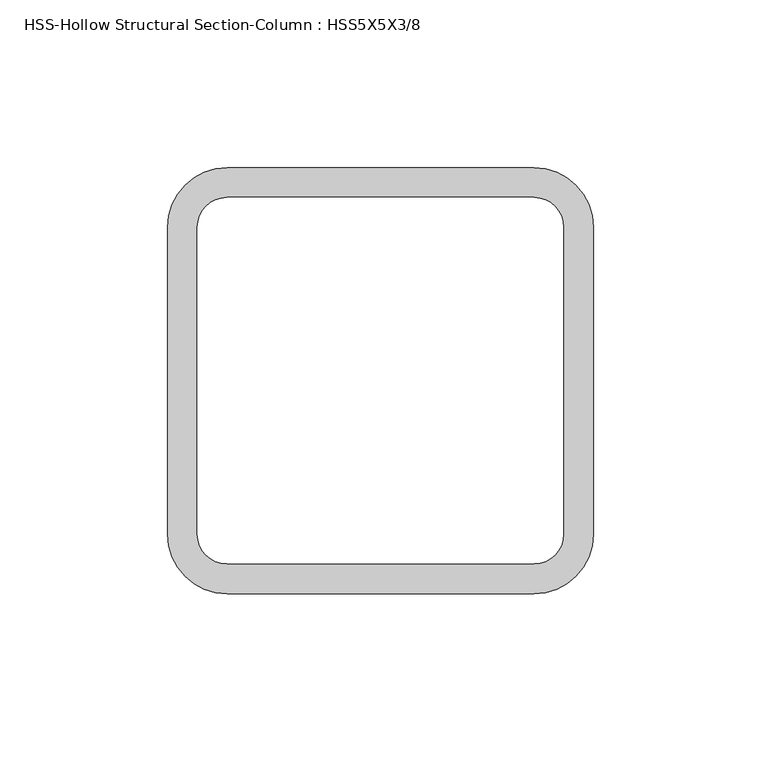
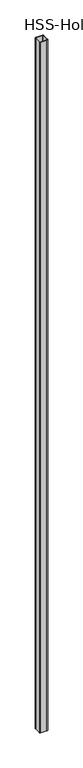
"""IFC4 building model written with IfcOpenShell, lengths in millimetres: column geometry, HSS-Hollow Structural Section-Column : HSS5X5X3/8."""

import ifcopenshell
import ifcopenshell.guid

model = None  # the IFC model being written
_history = None  # IfcOwnerHistory: only IFC2X3 demands one
_inside = {}  # id of a spatial element -> (the spatial element, [elements in it])
_under = {}  # id of a project, library or spatial element -> (it, [spatial elements below it])
_declared = {}  # id of a project -> (the project, [libraries it declares])
_typed = {}  # id of a type object -> (the type object, [elements of that type])
_made_of = {}  # id of a material, layer set ... -> (it, [elements and type objects made of it])


def new_model(schema):
    """Start an empty IFC model of exactly this schema.

    Asked for "IFC4X3", IfcOpenShell would pick the latest addendum, in which some entities
    have other attributes; the version numbers below select the first issue.
    IFC2X3 requires an IfcOwnerHistory on every rooted entity: one is made here for all.
    """
    global model, _history
    if schema == "IFC4X3":
        model = ifcopenshell.file(schema_version=(4, 3, 0, 0))
    else:
        model = ifcopenshell.file(schema=schema)
    _inside.clear()
    _under.clear()
    _declared.clear()
    _typed.clear()
    _made_of.clear()
    _history = None
    if model.schema == "IFC2X3":
        org = make("IfcOrganization", Name="unknown")
        user = make(
            "IfcPersonAndOrganization",
            ThePerson=make("IfcPerson", FamilyName="unknown"),
            TheOrganization=org,
        )
        app = make(
            "IfcApplication",
            ApplicationDeveloper=org,
            Version="unknown",
            ApplicationFullName="unknown",
            ApplicationIdentifier="unknown",
        )
        _history = make(
            "IfcOwnerHistory",
            OwningUser=user,
            OwningApplication=app,
            ChangeAction="ADDED",
            CreationDate=0,
        )
    return model


def make(cls, **values):
    """One entity of the class cls with the attributes given. An attribute that is None is left unset."""
    return model.create_entity(
        cls, **{name: value for name, value in values.items() if value is not None}
    )


def rooted(cls, **values):
    """An entity with a GlobalId (a new one), such as an element, a storey or a relation."""
    return make(cls, GlobalId=ifcopenshell.guid.new(), OwnerHistory=_history, **values)


def si_unit(unit_type, name, prefix=None):
    """IfcSIUnit, for example si_unit("LENGTHUNIT", "METRE", prefix="MILLI")."""
    return make("IfcSIUnit", UnitType=unit_type, Prefix=prefix, Name=name)


def assignment(units):
    """IfcUnitAssignment: the units of a project."""
    return None if units is None else make("IfcUnitAssignment", Units=units)


def point(xyz):
    """IfcCartesianPoint."""
    return None if xyz is None else make("IfcCartesianPoint", Coordinates=xyz)


def direction(xyz):
    """IfcDirection."""
    return None if xyz is None else make("IfcDirection", DirectionRatios=xyz)


def frame(location, z_axis=None, x_axis=None):
    """IfcAxis2Placement3D, a coordinate frame: its origin and axes. An axis left out is left unset."""
    return make(
        "IfcAxis2Placement3D",
        Location=point(location),
        Axis=direction(z_axis),
        RefDirection=direction(x_axis),
    )


def frame_2d(location, x_axis=None):
    """IfcAxis2Placement2D, a coordinate frame in the plane: its origin and x axis."""
    return make(
        "IfcAxis2Placement2D", Location=point(location), RefDirection=direction(x_axis)
    )


def origin():
    """The frame at (0, 0, 0) with its axes left unset."""
    return frame((0.0, 0.0, 0.0))


def place(relative_to, where):
    """IfcLocalPlacement: puts the frame where relative to a parent placement (None: the world)."""
    return make(
        "IfcLocalPlacement", PlacementRelTo=relative_to, RelativePlacement=where
    )


def context(
    kind, dimensions, precision=None, world=None, true_north=None, identifier=None
):
    """IfcGeometricRepresentationContext, for example the 3D "Model" context."""
    return make(
        "IfcGeometricRepresentationContext",
        ContextIdentifier=identifier,
        ContextType=kind,
        CoordinateSpaceDimension=dimensions,
        Precision=precision,
        WorldCoordinateSystem=world,
        TrueNorth=true_north,
    )


def project(units=None, contexts=None):
    """IfcProject with its units and contexts."""
    return rooted(
        "IfcProject",
        Name="project",
        RepresentationContexts=contexts,
        UnitsInContext=assignment(units),
    )


def spatial(cls, under=None, at=None, **own):
    """A site, building, storey or space (cls), placed at a placement, below another one or the project."""
    s = rooted(cls, ObjectPlacement=at, **own)
    if under is not None:
        _under.setdefault(under.id(), (under, []))[1].append(s)
    return s


def polyline(points):
    """IfcPolyline through the points."""
    return make("IfcPolyline", Points=[point(p) for p in points])


def circle_curve(where, radius):
    """IfcCircle in the frame where."""
    return make("IfcCircle", Position=where, Radius=radius)


def trimmed(basis, trim1, trim2, sense, master):
    """IfcTrimmedCurve: the piece of a basis curve between two trims."""
    return make(
        "IfcTrimmedCurve",
        BasisCurve=basis,
        Trim1=trim1,
        Trim2=trim2,
        SenseAgreement=sense,
        MasterRepresentation=master,
    )


def segment(curve, same_sense, transition):
    """IfcCompositeCurveSegment."""
    return make(
        "IfcCompositeCurveSegment",
        Transition=transition,
        SameSense=same_sense,
        ParentCurve=curve,
    )


def composite_curve(segments, self_intersect=None):
    """IfcCompositeCurve: segments joined end to end."""
    return make("IfcCompositeCurve", Segments=segments, SelfIntersect=self_intersect)


def outline(outer, holes=None, kind="AREA"):
    """IfcArbitraryClosedProfileDef: a profile drawn as a closed curve; with holes, ...WithVoids."""
    if holes is None:
        return make("IfcArbitraryClosedProfileDef", ProfileType=kind, OuterCurve=outer)
    return make(
        "IfcArbitraryProfileDefWithVoids",
        ProfileType=kind,
        OuterCurve=outer,
        InnerCurves=holes,
    )


def extrude(swept, where, along, depth):
    """IfcExtrudedAreaSolid: the profile swept, set in the frame where, extruded along a direction by depth."""
    return make(
        "IfcExtrudedAreaSolid",
        SweptArea=swept,
        Position=where,
        ExtrudedDirection=direction(along),
        Depth=depth,
    )


def shape(context_of_items, identifier, shape_type, items):
    """IfcShapeRepresentation: the items that make up one representation, for example the "Body"."""
    return make(
        "IfcShapeRepresentation",
        ContextOfItems=context_of_items,
        RepresentationIdentifier=identifier,
        RepresentationType=shape_type,
        Items=items,
    )


def source(mapping_origin, context_of_items, identifier, shape_type, items):
    """IfcRepresentationMap: a shape defined once, which mapped items show again and again."""
    return make(
        "IfcRepresentationMap",
        MappingOrigin=mapping_origin,
        MappedRepresentation=shape(context_of_items, identifier, shape_type, items),
    )


def transform(
    local_origin,
    x_axis=None,
    y_axis=None,
    z_axis=None,
    scale=None,
    scale2=None,
    scale3=None,
    uniform=True,
):
    """IfcCartesianTransformationOperator3D, or its non-uniform kind. x_axis, y_axis, z_axis: its Axis1, 2, 3."""
    if uniform:
        return make(
            "IfcCartesianTransformationOperator3D",
            Axis1=direction(x_axis),
            Axis2=direction(y_axis),
            LocalOrigin=point(local_origin),
            Scale=scale,
            Axis3=direction(z_axis),
        )
    return make(
        "IfcCartesianTransformationOperator3DnonUniform",
        Axis1=direction(x_axis),
        Axis2=direction(y_axis),
        LocalOrigin=point(local_origin),
        Scale=scale,
        Axis3=direction(z_axis),
        Scale2=scale2,
        Scale3=scale3,
    )


def mapped(mapping_source, mapping_target):
    """IfcMappedItem: shows the shape of a source again, moved by a transform."""
    return make(
        "IfcMappedItem", MappingSource=mapping_source, MappingTarget=mapping_target
    )


def made_of(thing, what):
    """Note that an element or type object is made of a material, layer set ...; save() writes the relation."""
    if what is not None:
        _made_of.setdefault(what.id(), (what, []))[1].append(thing)
    return thing


def element(
    cls,
    number,
    at=None,
    inside=None,
    cuts=None,
    type_object=None,
    material=None,
    context=None,
    identifier="Body",
    shape_type=None,
    held_by="IfcProductDefinitionShape",
    body=None,
    shapes=None,
    **own,
):
    """One element of the class cls, such as IfcWall. Its Tag is "e" and its number.

    at: its placement. inside: the storey or other place that contains it. cuts: it is an
    opening in that element (IfcRelVoidsElement). A single representation is given by context,
    identifier, shape_type and body (its items); several are given by shapes. held_by: the class
    of the entity that holds the representations. save() writes the other relations.
    """
    e = rooted(cls, Tag="e%d" % number, ObjectPlacement=at, **own)
    if body is not None:
        shapes = [shape(context, identifier, shape_type, body)]
    if shapes is not None:
        e.Representation = make(held_by, Representations=shapes)
    if inside is not None:
        _inside.setdefault(inside.id(), (inside, []))[1].append(e)
    if cuts is not None:
        rooted(
            "IfcRelVoidsElement", RelatingBuildingElement=cuts, RelatedOpeningElement=e
        )
    if type_object is not None:
        _typed.setdefault(type_object.id(), (type_object, []))[1].append(e)
    return made_of(e, material)


def aggregate(whole, parts):
    """IfcRelAggregates: a whole, such as a stair, and the parts it consists of."""
    return rooted("IfcRelAggregates", RelatingObject=whole, RelatedObjects=parts)


def save(model, path):
    """Write the relations noted so far, then the file.

    IfcRelAggregates (storeys below a building ...), IfcRelContainedInSpatialStructure (elements
    in a storey), IfcRelDefinesByType, IfcRelAssociatesMaterial and IfcRelDeclares: one each for
    every whole, place, type object, material and project.
    """
    for whole, parts in _under.values():
        aggregate(whole, parts)
    for where, things in _inside.values():
        rooted(
            "IfcRelContainedInSpatialStructure",
            RelatedElements=things,
            RelatingStructure=where,
        )
    for kind, things in _typed.values():
        rooted("IfcRelDefinesByType", RelatedObjects=things, RelatingType=kind)
    for what, things in _made_of.values():
        rooted("IfcRelAssociatesMaterial", RelatedObjects=things, RelatingMaterial=what)
    for by, libraries in _declared.values():
        rooted("IfcRelDeclares", RelatingContext=by, RelatedDefinitions=libraries)
    model.write(path)


def hss_hollow_structural_section_column_hss5x5x3_8_a8b47676(model_context):
    return source(origin(), model_context, "Body", "SweptSolid", [
        extrude(outline(composite_curve([segment(trimmed(circle_curve(frame_2d((45.7708, 45.7708)), 17.7292), [point((45.7708, 63.5))], [point((63.5, 45.7708))], False, "CARTESIAN"), True, "CONTINUOUS"), segment(polyline([(63.5, 45.7708), (63.5, -45.7708)]), True, "CONTINUOUS"), segment(trimmed(circle_curve(frame_2d((45.7708, -45.7708)), 17.7292), [point((63.5, -45.7708))], [point((45.7708, -63.5))], False, "CARTESIAN"), True, "CONTINUOUS"), segment(polyline([(45.7708, -63.5), (-45.7708, -63.5)]), True, "CONTINUOUS"), segment(trimmed(circle_curve(frame_2d((-45.7708, -45.7708)), 17.7292), [point((-45.7708, -63.5))], [point((-63.5, -45.7708))], False, "CARTESIAN"), True, "CONTINUOUS"), segment(polyline([(-63.5, -45.7708), (-63.5, 45.7708)]), True, "CONTINUOUS"), segment(trimmed(circle_curve(frame_2d((-45.7708, 45.7708)), 17.7292), [point((-63.5, 45.7708))], [point((-45.7708, 63.5))], False, "CARTESIAN"), True, "CONTINUOUS"), segment(polyline([(-45.7708, 63.5), (45.7708, 63.5)]), True, "CONTINUOUS")], self_intersect=False), holes=[composite_curve([segment(polyline([(45.7708, 54.6354), (-45.7708, 54.6354)]), True, "CONTINUOUS"), segment(trimmed(circle_curve(frame_2d((-45.7708, 45.7708)), 8.8646), [point((-45.7708, 54.6354))], [point((-54.6354, 45.7708))], True, "CARTESIAN"), True, "CONTINUOUS"), segment(polyline([(-54.6354, 45.7708), (-54.6354, -45.7708)]), True, "CONTINUOUS"), segment(trimmed(circle_curve(frame_2d((-45.7708, -45.7708)), 8.8646), [point((-54.6354, -45.7708))], [point((-45.7708, -54.6354))], True, "CARTESIAN"), True, "CONTINUOUS"), segment(polyline([(-45.7708, -54.6354), (45.7708, -54.6354)]), True, "CONTINUOUS"), segment(trimmed(circle_curve(frame_2d((45.7708, -45.7708)), 8.8646), [point((45.7708, -54.6354))], [point((54.6354, -45.7708))], True, "CARTESIAN"), True, "CONTINUOUS"), segment(polyline([(54.6354, -45.7708), (54.6354, 45.7708)]), True, "CONTINUOUS"), segment(trimmed(circle_curve(frame_2d((45.7708, 45.7708)), 8.8646), [point((54.6354, 45.7708))], [point((45.7708, 54.6354))], True, "CARTESIAN"), True, "CONTINUOUS")], self_intersect=False)]), frame((0.0, 0.0, 16408.4), z_axis=(0.0, 0.0, 1.0), x_axis=(1.0, 0.0, 0.0)), (0.0, 0.0, 1.0), 11176.0),
    ])


if __name__ == "__main__":
    model = new_model("IFC4")
    model_context = context("Model", 3, world=origin())
    ifc_project = project(units=[si_unit("LENGTHUNIT", "METRE", prefix="MILLI")], contexts=[model_context])
    site = spatial("IfcSite", under=ifc_project)
    building = spatial("IfcBuilding", under=site)
    placement = place(None, origin())
    hss_hollow_structural_section_column_hss5x5x3_8_shape = hss_hollow_structural_section_column_hss5x5x3_8_a8b47676(model_context)
    element("IfcColumn", 1, ObjectType="HSS-Hollow Structural Section-Column : HSS5X5X3/8", at=placement, inside=building, context=model_context, shape_type="MappedRepresentation", body=[
        mapped(hss_hollow_structural_section_column_hss5x5x3_8_shape, transform((0.0, 0.0, 0.0), x_axis=(1.0, 0.0, 0.0), y_axis=(0.0, 1.0, 0.0), z_axis=(0.0, 0.0, 1.0))),
    ])
    save(model, "model.ifc")

# Revit data of these elements
# Type "HSS-Hollow Structural Section-Column : HSS5X5X3/8"
#   Assembly Code = "B10"
#   Shape = "Square"
#   W = 22.3
#   Ht = 0' - 5"
#   b = 0' - 5"
#   kr = 0' - 0.698"
#   t = 0' - 0.349"
#   A = 0.0429167 SF
#   Structural Material [instance default] = Steel ASTM A500, Grade B, Rectangular and Square
# Element 1 (IfcColumn, "HSS-Hollow Structural Section-Column : HSS5X5X3/8")
#   Materials on its faces: "Steel ASTM A500, Grade B, Rectangular and Square"
# Materials
#   "Steel ASTM A500, Grade B, Rectangular and Square": class "Metal", colour RGB 199 199 199, transparency 0, Description = "Carbon steel", Cost = 0
